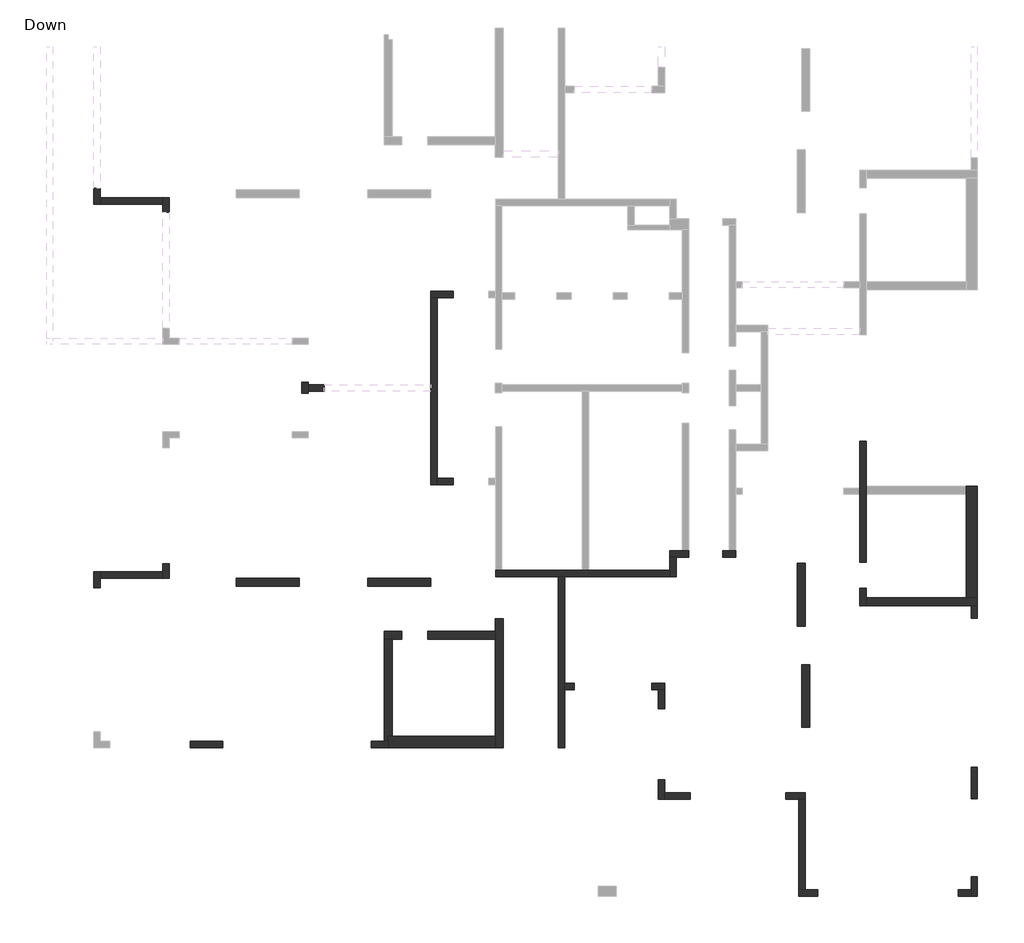
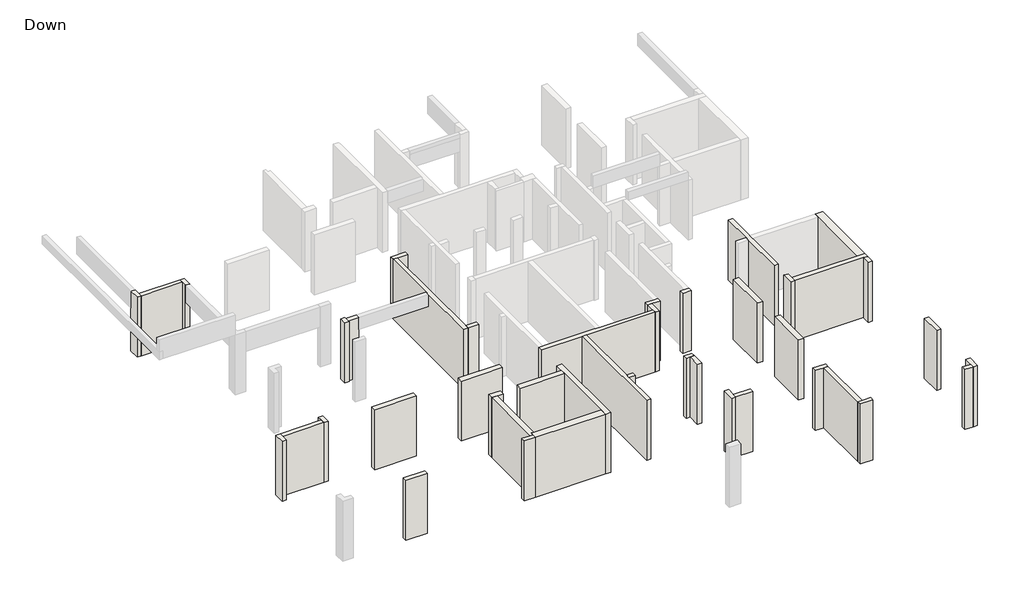
# One storey, part 1 of 3: 43 walls.
# Revit data of these elements (continued)
# Element 40 (IfcWall, "25") (continued)
#   SOFiSTiK_EdgeZones = "W104"
#   SOFiSTiK_AMG_Comments = ""
#   Top Offset = 0 cm
#   Base Offset = 0 cm
#   wall height = 300 cm
#   SOFiSTiK_AMG_Scheduled = yes
#   SOFiSTiK_AMG_Adjusted = yes
#   Phase Created = New Construction
#   Base Constraint = Down
#   Top Constraint = Typical Floor
#   Materials on its faces: "Concrete"
# Element 41 (IfcWall, "25")
#   Comments = ""
#   Mark = "W105"
#   SOFiSTiK_EdgeZones = "W105"
#   SOFiSTiK_AMG_Comments = ""
#   Top Offset = 0 cm
#   Base Offset = 0 cm
#   wall height = 300 cm
#   SOFiSTiK_AMG_Scheduled = yes
#   SOFiSTiK_AMG_Adjusted = yes
#   Phase Created = New Construction
#   Base Constraint = Down
#   Top Constraint = Typical Floor
#   Materials on its faces: "Concrete"
# Element 42 (IfcWall, "35")
#   Comments = ""
#   Mark = "W110"
#   SOFiSTiK_EdgeZones = "W110"
#   SOFiSTiK_AMG_Comments = ""
#   Top Offset = 0 cm
#   Base Offset = 0 cm
#   wall height = 300 cm
#   SOFiSTiK_AMG_Scheduled = yes
#   SOFiSTiK_AMG_Adjusted = yes
#   Phase Created = New Construction
#   Base Constraint = Down
#   Top Constraint = Typical Floor
#   Materials on its faces: "Concrete"
# Element 43 (IfcWall, "35")
#   Comments = ""
#   Mark = "W111"
#   SOFiSTiK_EdgeZones = "W111"
#   SOFiSTiK_AMG_Comments = ""
#   Top Offset = 0 cm
#   Base Offset = 0 cm
#   wall height = 300 cm
#   SOFiSTiK_AMG_Scheduled = yes
#   SOFiSTiK_AMG_Adjusted = yes
#   Phase Created = New Construction
#   Base Constraint = Down
#   Top Constraint = Typical Floor
#   Materials on its faces: "Concrete"
# Materials
#   "Concrete": class "Concrete", colour RGB 192 192 192, transparency 0, Keynote = "01000", Description = "Cast-in-place concrete", Cost = 0
